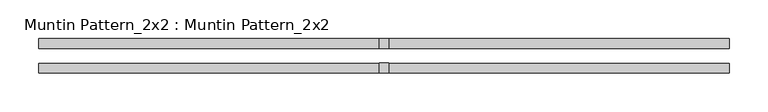
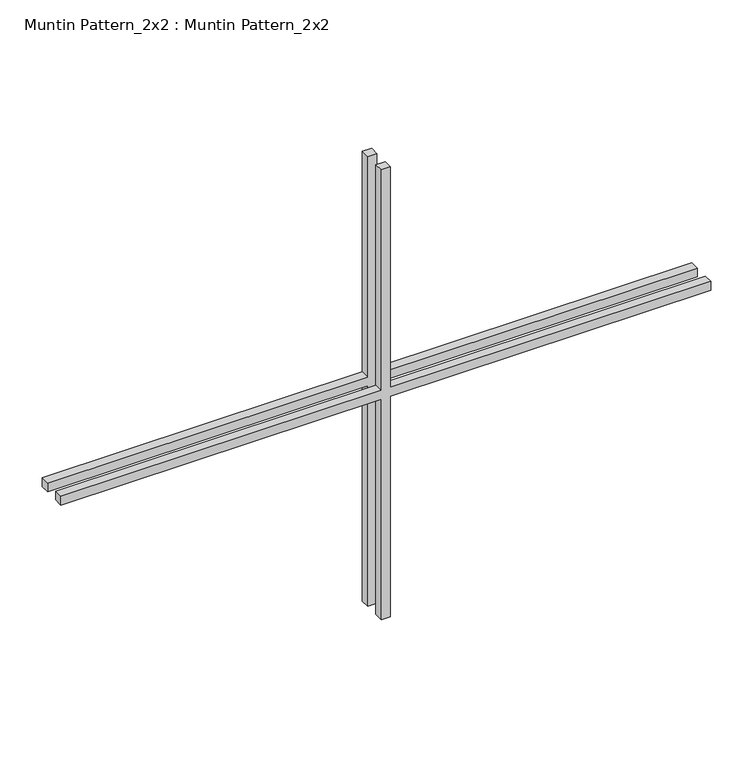
"""IFC4 building model written with IfcOpenShell, lengths in millimetres: proxy geometry, Muntin Pattern_2x2 : Muntin Pattern_2x2."""

from ifc_helpers import new_model, si_unit, frame, origin, place, context, project, spatial, polyline, outline, extrude, source, transform, mapped, element, save


def muntin_pattern_2x2_muntin_pattern_2x2_9281f183(model_context):
    return source(origin(), model_context, "Body", "SweptSolid", [
        extrude(outline(polyline([(331.7875, -6.35), (331.7875, -444.5), (319.0875, -444.5), (319.0875, -6.35), (0.0, -6.35), (0.0, 6.35), (319.0875, 6.35), (319.0875, 444.5), (331.7875, 444.5), (331.7875, 6.35), (650.875, 6.35), (650.875, -6.35), (331.7875, -6.35)])), frame((0.0, 9.525, 0.0), z_axis=(0.0, 1.0, 0.0), x_axis=(0.0, 0.0, 1.0)), (0.0, 0.0, 1.0), 12.7),
        extrude(outline(polyline([(331.7875, -6.35), (331.7875, -444.5), (319.0875, -444.5), (319.0875, -6.35), (0.0, -6.35), (0.0, 6.35), (319.0875, 6.35), (319.0875, 444.5), (331.7875, 444.5), (331.7875, 6.35), (650.875, 6.35), (650.875, -6.35), (331.7875, -6.35)])), frame((0.0, -22.225, 0.0), z_axis=(0.0, 1.0, 0.0), x_axis=(0.0, 0.0, 1.0)), (0.0, 0.0, 1.0), 12.7),
    ])


if __name__ == "__main__":
    model = new_model("IFC4")
    model_context = context("Model", 3, world=origin())
    ifc_project = project(units=[si_unit("LENGTHUNIT", "METRE", prefix="MILLI")], contexts=[model_context])
    site = spatial("IfcSite", under=ifc_project)
    building = spatial("IfcBuilding", under=site)
    placement = place(None, origin())
    muntin_pattern_2x2_muntin_pattern_2x2_shape = muntin_pattern_2x2_muntin_pattern_2x2_9281f183(model_context)
    element("IfcBuildingElementProxy", 1, Name="Muntin Pattern_2x2 : Muntin Pattern_2x2", ObjectType="Muntin Pattern_2x2 : Muntin Pattern_2x2", at=placement, inside=building, context=model_context, shape_type="MappedRepresentation", body=[
        mapped(muntin_pattern_2x2_muntin_pattern_2x2_shape, transform((0.0, 0.0, 0.0), x_axis=(1.0, 0.0, 0.0), y_axis=(0.0, 1.0, 0.0), z_axis=(0.0, 0.0, 1.0))),
    ])
    save(model, "model.ifc")

# Revit data of these elements
# Type "Muntin Pattern_2x2 : Muntin Pattern_2x2"
#   Width [instance default] = 4' - 0"
#   Thickness = 0' - 0 1/2"
#   Height [instance default] = 4' - 0"
#   Distance = 0' - 0 3/4"
#   Interior Material [instance default] = none
#   Exterior Material [instance default] = none
# Element 1 (IfcBuildingElementProxy, "Muntin Pattern_2x2 : Muntin Pattern_2x2")
#   Width = 2' - 11"
#   Height = 2' - 1 5/8"
#   Interior Material = Wood - Stained
#   Exterior Material = Clad - White
#   Materials on its faces: "Clad - White", "Wood - Stained"
# Materials
#   "Clad - White": class "Wood", colour RGB 242 242 238, transparency 0, Cost = 0
#   "Wood - Stained": class "Wood", colour RGB 224 178 126, transparency 0, Cost = 0
